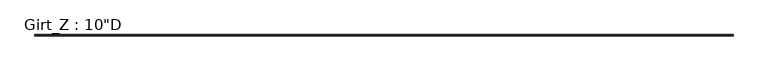
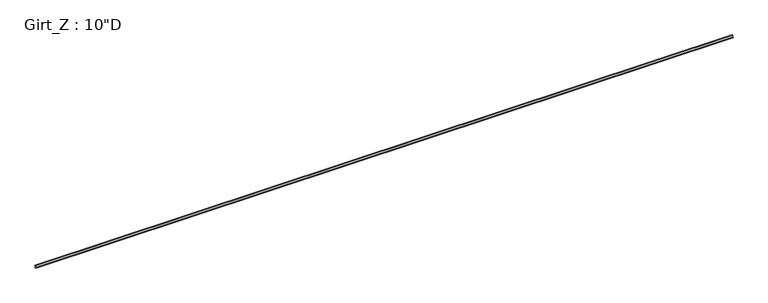
"""IFC4 building model written with IfcOpenShell, lengths in millimetres: beam geometry."""

from ifc_helpers import new_model, si_unit, point, frame, frame_2d, origin, place, context, project, spatial, polyline, circle_curve, trimmed, segment, composite_curve, outline, extrude, source, transform, mapped, element, save


def beam_c5090da8(model_context):
    return source(origin(), model_context, "Body", "SweptSolid", [
        extrude(outline(composite_curve([segment(polyline([(77.9859375, 127.0), (90.2310415, 112.4068534), (88.1028742, 110.621109), (76.6904765, 124.221875), (3.3005807, 124.221875)]), True, "CONTINUOUS"), segment(trimmed(circle_curve(frame_2d((3.3741066, 122.2381931)), 1.9850441), [point((3.3005807, 124.221875))], [point((1.3890625, 122.2381931))], True, "CARTESIAN"), True, "CONTINUOUS"), segment(polyline([(1.3890625, 122.2381931), (1.3890625, -127.0), (-84.3359375, -127.0), (-96.5810415, -112.4068534), (-94.4528742, -110.621109), (-83.0404765, -124.221875), (-3.2694106, -124.221875)]), True, "CONTINUOUS"), segment(trimmed(circle_curve(frame_2d((-3.3748024, -122.2389339)), 1.9857399), [point((-3.2694106, -124.221875))], [point((-1.3890625, -122.2389339))], True, "CARTESIAN"), True, "CONTINUOUS"), segment(polyline([(-1.3890625, -122.2389339), (-1.3890625, 122.2375)]), True, "CONTINUOUS"), segment(trimmed(circle_curve(frame_2d((3.3734375, 122.2375)), 4.7625), [point((-1.3890625, 122.2375))], [point((3.3734375, 127.0))], False, "CARTESIAN"), True, "CONTINUOUS"), segment(polyline([(3.3734375, 127.0), (77.9859375, 127.0)]), True, "CONTINUOUS")], self_intersect=False)), frame((-43981.290625, 0.0, 0.0), z_axis=(1.0, 0.0, 0.0), x_axis=(0.0, 1.0, 0.0)), (0.0, 0.0, 1.0), 88138.0),
    ])


if __name__ == "__main__":
    model = new_model("IFC4")
    model_context = context("Model", 3, world=origin())
    ifc_project = project(units=[si_unit("LENGTHUNIT", "METRE", prefix="MILLI")], contexts=[model_context])
    site = spatial("IfcSite", under=ifc_project)
    building = spatial("IfcBuilding", under=site)
    placement = place(None, origin())
    beam_shape = beam_c5090da8(model_context)
    element("IfcBeam", 1, ObjectType="Girt_Z : 10\"D", at=placement, inside=building, context=model_context, shape_type="MappedRepresentation", body=[
        mapped(beam_shape, transform((0.0, 0.0, 0.0), x_axis=(1.0, 0.0, 0.0), y_axis=(0.0, 1.0, 0.0), z_axis=(0.0, 0.0, 1.0))),
    ])
    save(model, "model.ifc")

# Revit data of these elements
# Type "Girt_Z : 10\"D"
#   half leg = 0' - 1 11/16"
#   Web_Thickness = 0' - 0 7/64"
#   Length [instance default] = 10' - 0"
#   Leg_2 = 0' - 3 3/8"
#   Leg_1 = 0' - 3 1/8"
#   Height = 0' - 10"
#   Structural Material [instance default] = none
